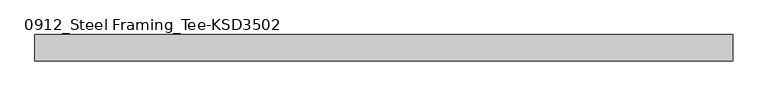
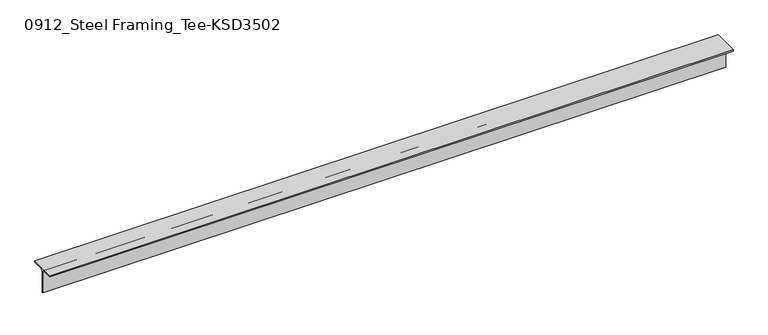
"""IFC4 building model written with IfcOpenShell, lengths in millimetres: member geometry, 0912_Steel Framing_Tee-KSD3502 : H_SB_ASB_CT-150x150x6.5x9."""

from ifc_helpers import new_model, si_unit, point, frame, frame_2d, origin, place, context, project, spatial, polyline, circle_curve, trimmed, segment, composite_curve, outline, extrude, source, transform, mapped, element, save


def member_0912_steel_framing_tee_ksd3502_48611037(model_context):
    return source(origin(), model_context, "Body", "SweptSolid", [
        extrude(outline(composite_curve([segment(polyline([(-75.0, 75.0), (75.0, 75.0), (75.0, 66.0), (16.25, 66.0)]), True, "CONTINUOUS"), segment(trimmed(circle_curve(frame_2d((16.25, 53.0)), 13.0), [point((16.25, 66.0))], [point((3.25, 53.0))], True, "CARTESIAN"), True, "CONTINUOUS"), segment(polyline([(3.25, 53.0), (3.25, -75.0), (-3.25, -75.0), (-3.25, 53.0)]), True, "CONTINUOUS"), segment(trimmed(circle_curve(frame_2d((-16.25, 53.0)), 13.0), [point((-3.25, 53.0))], [point((-16.25, 66.0))], True, "CARTESIAN"), True, "CONTINUOUS"), segment(polyline([(-16.25, 66.0), (-75.0, 66.0), (-75.0, 75.0)]), True, "CONTINUOUS")], self_intersect=False)), frame((-1988.55, 0.0, 0.0), z_axis=(1.0, 0.0, 0.0), x_axis=(0.0, 1.0, 0.0)), (0.0, 0.0, 1.0), 3954.0),
    ])


if __name__ == "__main__":
    model = new_model("IFC4")
    model_context = context("Model", 3, world=origin())
    ifc_project = project(units=[si_unit("LENGTHUNIT", "METRE", prefix="MILLI")], contexts=[model_context])
    site = spatial("IfcSite", under=ifc_project)
    building = spatial("IfcBuilding", under=site)
    placement = place(None, origin())
    member_0912_steel_framing_tee_ksd3502_shape = member_0912_steel_framing_tee_ksd3502_48611037(model_context)
    element("IfcMember", 1, ObjectType="0912_Steel Framing_Tee-KSD3502 : H_SB_ASB_CT-150x150x6.5x9", at=placement, inside=building, context=model_context, shape_type="MappedRepresentation", body=[
        mapped(member_0912_steel_framing_tee_ksd3502_shape, transform((0.0, 0.0, 0.0), x_axis=(1.0, 0.0, 0.0), y_axis=(0.0, 1.0, 0.0), z_axis=(0.0, 0.0, 1.0))),
    ])
    save(model, "model.ifc")

# Revit data of these elements
# Type "0912_Steel Framing_Tee-KSD3502 : H_SB_ASB_CT-150x150x6.5x9"
#   H_WM Code_1 = "S01AA003-00001 | Main Steel Structure Fabrication Work | Shelter/Building | Light Steel - Standard (30KG/M>Weight) | Material: (   )"
#   H_WM Code_2 = "S03AA029-00001 | Main Steel Structure Erection Work | Shelter/Building | Light Steel (30KG/M>Weight) | Material: (   )"
#   H_WM Code_3 = "S01AA010-00001 | Main Steel Structure Fabrication Work | Shelter/Building | Steel Painting/Coating | for Non-Fireproofed Steel Surface, Surface Preparation, Primer, Second & Final Coat | Material: (   )"
#   H_Q'ty Cal Type Tag = "SB-Q2"
#   Width = 15.0 cm
#   Web Thickness = 0.65 cm
#   Web Fillet = 1.3 cm
#   Section Area = 23.39 cm²
#   Perimeter = 0.60 m²/m
#   Nominal Weight = 18.40 kgf/m
#   Height = 15.0 cm
#   Flange Thickness = 0.9 cm
#   Centroid Vertical = 7.5 cm
#   Centroid Horizontal = 7.5 cm
#   Length [instance default] = 1.5000 m
#   Structural Material [instance default] = Steel, 45-345
#   Warping Constant = (empty or 0)
#   Torsional Moment of Inertia = 0
#   Section Name Key = ""
#   Plastic Modulus weak axis = 0
#   Plastic Modulus strong axis = 0
#   Moment of Inertia weak axis = 0
#   Moment of Inertia strong axis = 0
#   Elastic Modulus weak axis = 0
#   Elastic Modulus strong axis = 0
#   Bolt Spacing = 0
#   Assembly Code = ""
# Element 1 (IfcMember, "0912_Steel Framing_Tee-KSD3502 : H_SB_ASB_CT-150x150x6.5x9")
#   Structural Material = none
# Materials
#   "Steel, 45-345": class "Metal", colour RGB 189 187 185, transparency 0, Description = "Steel 345 MPa", Cost = 0
